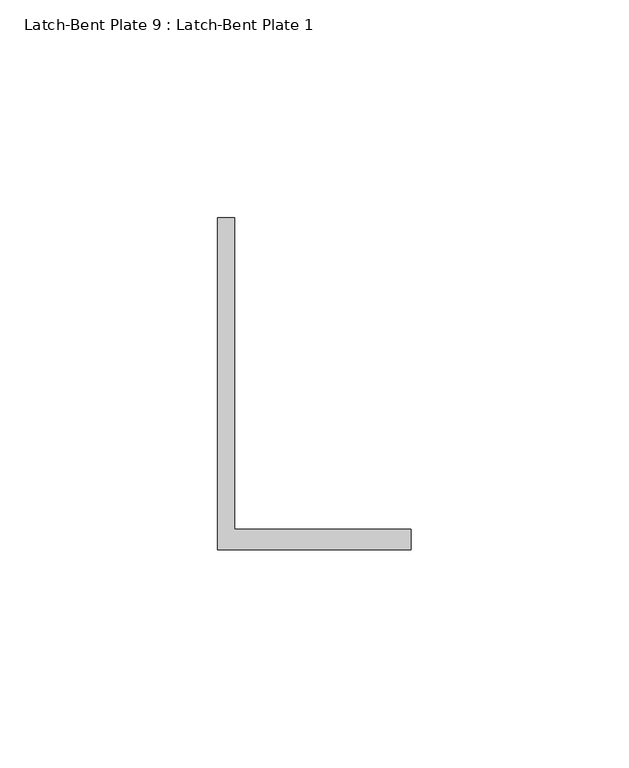
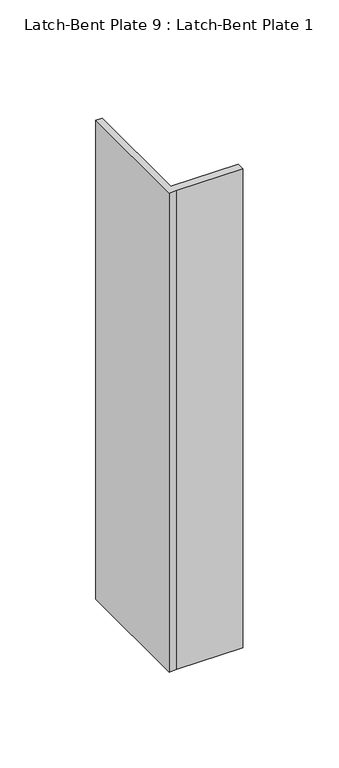
"""IFC4 building model written with IfcOpenShell, lengths in millimetres: proxy geometry, Latch-Bent Plate 9 : Latch-Bent Plate 1."""

from ifc_helpers import new_model, si_unit, frame, origin, place, context, project, spatial, polyline, outline, extrude, source, transform, mapped, element, save


def latch_bent_plate_9_latch_bent_plate_1_ca46e00b(model_context):
    return source(origin(), model_context, "Body", "SweptSolid", [
        extrude(outline(polyline([(587327.0060739, -532877.4663841), (587322.2435739, -532877.4663841), (587322.2435739, -532801.2663841), (587326.1141748, -532801.2663841), (587326.1141748, -532872.7038841), (587366.6808739, -532872.7038841), (587366.6808739, -532877.4663841), (587327.0060739, -532877.4663841)])), frame((0.0, 0.0, 50.8), z_axis=(0.0, 0.0, 1.0), x_axis=(1.0, 0.0, 0.0)), (0.0, 0.0, 1.0), 304.8),
    ])


if __name__ == "__main__":
    model = new_model("IFC4")
    model_context = context("Model", 3, world=origin())
    ifc_project = project(units=[si_unit("LENGTHUNIT", "METRE", prefix="MILLI")], contexts=[model_context])
    site = spatial("IfcSite", under=ifc_project)
    building = spatial("IfcBuilding", under=site)
    placement = place(None, origin())
    latch_bent_plate_9_latch_bent_plate_1_shape = latch_bent_plate_9_latch_bent_plate_1_ca46e00b(model_context)
    element("IfcBuildingElementProxy", 1, Name="Latch-Bent Plate 9 : Latch-Bent Plate 1", ObjectType="Latch-Bent Plate 9 : Latch-Bent Plate 1", at=placement, inside=building, context=model_context, shape_type="MappedRepresentation", body=[
        mapped(latch_bent_plate_9_latch_bent_plate_1_shape, transform((0.0, 0.0, 0.0), x_axis=(1.0, 0.0, 0.0), y_axis=(0.0, 1.0, 0.0), z_axis=(0.0, 0.0, 1.0))),
    ])
    save(model, "model.ifc")

# Revit data of these elements
# Element 1 (IfcBuildingElementProxy, "Latch-Bent Plate 9 : Latch-Bent Plate 1")
#   Materials on its faces: "GALV. GATE LATCH"
# Materials
#   "GALV. GATE LATCH": class "Metal", colour RGB 189 187 185, transparency 0, Description = "Carbon steel", Cost = 0
